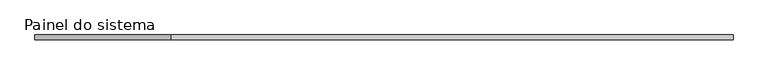
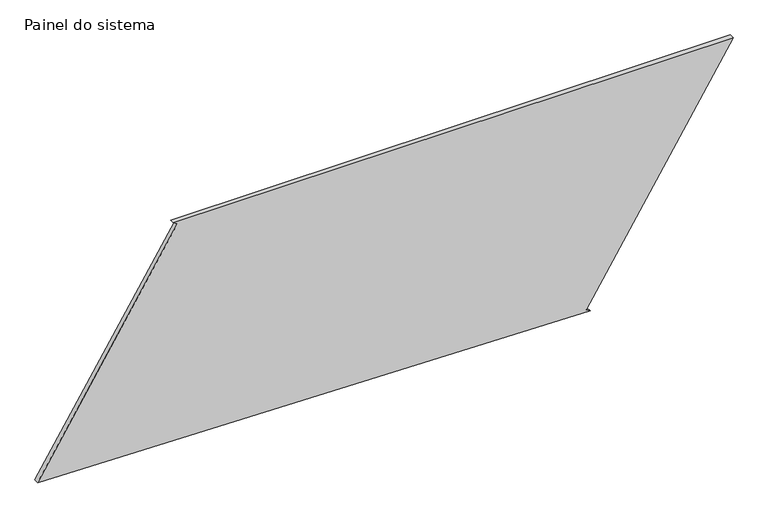
"""IFC4 building model written with IfcOpenShell, lengths in millimetres: plate geometry, Painel do sistema : Envidraçado."""

from ifc_helpers import new_model, si_unit, frame, origin, place, context, project, spatial, polyline, outline, extrude, source, transform, mapped, element, save


def painel_do_sistema_d52c9c95(model_context):
    return source(origin(), model_context, "Body", "SweptSolid", [
        extrude(outline(polyline([(0.0, 1097.5822541), (13.2016257, 1076.3521557), (1279.1523572, 1863.5650734), (1279.1523572, -1136.4550963), (1265.9507315, -1115.2249979), (62.5130787, -1863.5650734), (0.0, 1097.5822541)])), frame((0.0, 24.5, 0.0), z_axis=(0.0, 1.0, 0.0), x_axis=(0.0, 0.0, 1.0)), (0.0, 0.0, 1.0), 25.0),
    ])


if __name__ == "__main__":
    model = new_model("IFC4")
    model_context = context("Model", 3, world=origin())
    ifc_project = project(units=[si_unit("LENGTHUNIT", "METRE", prefix="MILLI")], contexts=[model_context])
    site = spatial("IfcSite", under=ifc_project)
    building = spatial("IfcBuilding", under=site)
    placement = place(None, origin())
    painel_do_sistema_shape = painel_do_sistema_d52c9c95(model_context)
    element("IfcPlate", 1, ObjectType="Painel do sistema : Envidraçado", at=placement, inside=building, context=model_context, shape_type="MappedRepresentation", body=[
        mapped(painel_do_sistema_shape, transform((0.0, 0.0, 0.0), x_axis=(1.0, 0.0, 0.0), y_axis=(0.0, 1.0, 0.0), z_axis=(0.0, 0.0, 1.0))),
    ])
    save(model, "model.ifc")

# Revit data of these elements
# Type "Painel do sistema : Envidraçado"
#   Construction Type Id = "GSP4R"
#   Analytic Construction = "Vidraça única Pilkington 1/8 pol"
#   Visual Light Transmittance = 0.9
#   Solar Heat Gain Coefficient = 0.86
#   Heat Transfer Coefficient (U) = 6.7069 W/(m²·K)
# Element 1 (IfcPlate, "Painel do sistema : Envidraçado")
#   Materials on its faces: "Vidro"
# Materials
#   "Vidro": class "Vidro", colour RGB 0 128 192, transparency 0.9, Description = "Vidro de sílica", Cost = 0
